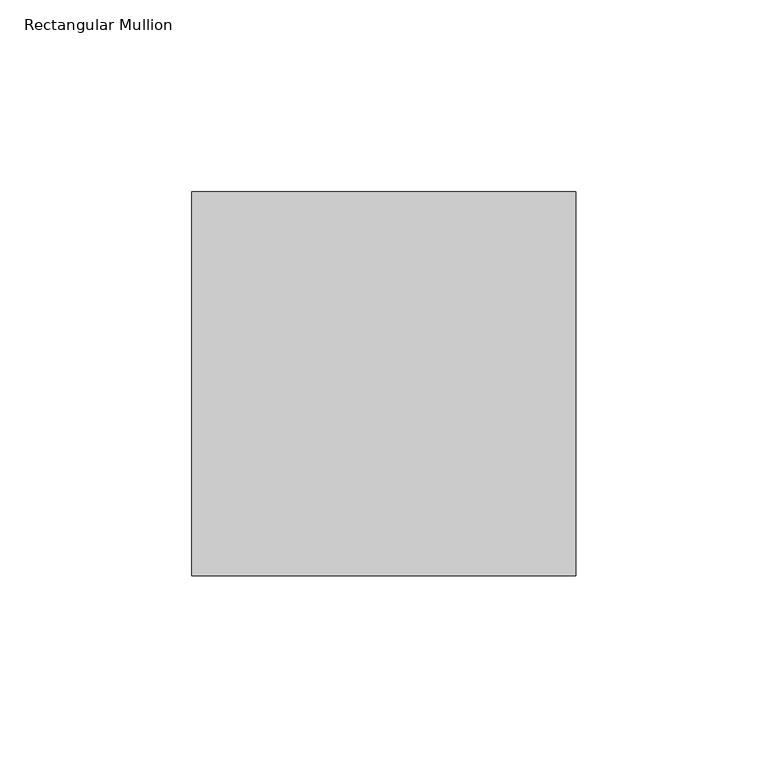
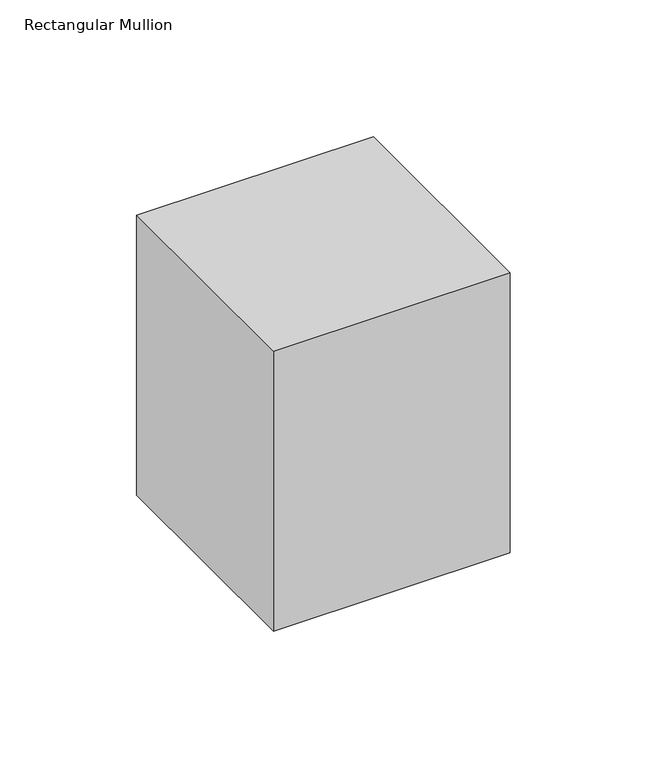
"""IFC4 building model written with IfcOpenShell, lengths in millimetres: member geometry, Rectangular Mullion : 알루미늄_Rectangular Cap_100 x100."""

from ifc_helpers import new_model, si_unit, frame, origin, place, context, project, spatial, polyline, outline, extrude, source, transform, mapped, element, save


def rectangular_mullion_9852de7d(model_context):
    return source(origin(), model_context, "Body", "SweptSolid", [
        extrude(outline(polyline([(0.0, 50.0), (0.0, -50.0), (-100.0, -50.0), (-100.0, 50.0), (0.0, 50.0)])), frame((0.0, 0.0, -125.0), z_axis=(0.0, 0.0, 1.0), x_axis=(1.0, 0.0, 0.0)), (0.0, 0.0, 1.0), 125.0),
    ])


if __name__ == "__main__":
    model = new_model("IFC4")
    model_context = context("Model", 3, world=origin())
    ifc_project = project(units=[si_unit("LENGTHUNIT", "METRE", prefix="MILLI")], contexts=[model_context])
    site = spatial("IfcSite", under=ifc_project)
    building = spatial("IfcBuilding", under=site)
    placement = place(None, origin())
    rectangular_mullion_shape = rectangular_mullion_9852de7d(model_context)
    element("IfcMember", 1, ObjectType="Rectangular Mullion : 알루미늄_Rectangular Cap_100 x100", at=placement, inside=building, context=model_context, shape_type="MappedRepresentation", body=[
        mapped(rectangular_mullion_shape, transform((0.0, 0.0, 0.0), x_axis=(1.0, 0.0, 0.0), y_axis=(0.0, 1.0, 0.0), z_axis=(0.0, 0.0, 1.0))),
    ])
    save(model, "model.ifc")

# Revit data of these elements
# Type "Rectangular Mullion : 알루미늄_Rectangular Cap_100 x100"
#   built-in parameter 1007304 = 0.328084 (stored number, unit not read)
#   built-in parameter 1007301 = 0.164042 (stored number, unit not read)
#   built-in parameter 1007300 = 0.164042 (stored number, unit not read)
# Element 1 (IfcMember, "Rectangular Mullion : 알루미늄_Rectangular Cap_100 x100")
#   Materials on its faces: "00_Metal_Stainless Steel"
# Materials
#   "00_Metal_Stainless Steel": class "Metal", colour RGB 148 148 148, transparency 0, Description = "Steel", Cost = 0
